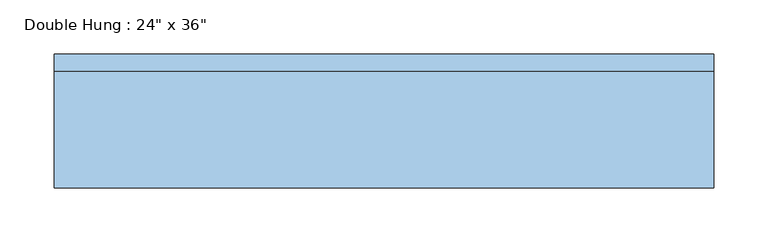
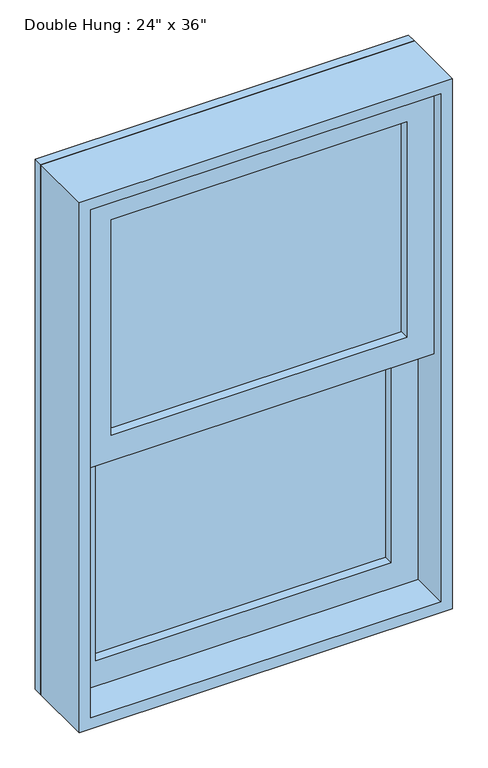
"""IFC4 building model written with IfcOpenShell, lengths in millimetres: window geometry."""

import ifcopenshell
import ifcopenshell.guid

model = None  # the IFC model being written
_history = None  # IfcOwnerHistory: only IFC2X3 demands one
_inside = {}  # id of a spatial element -> (the spatial element, [elements in it])
_under = {}  # id of a project, library or spatial element -> (it, [spatial elements below it])
_declared = {}  # id of a project -> (the project, [libraries it declares])
_typed = {}  # id of a type object -> (the type object, [elements of that type])
_made_of = {}  # id of a material, layer set ... -> (it, [elements and type objects made of it])


def new_model(schema):
    """Start an empty IFC model of exactly this schema.

    Asked for "IFC4X3", IfcOpenShell would pick the latest addendum, in which some entities
    have other attributes; the version numbers below select the first issue.
    IFC2X3 requires an IfcOwnerHistory on every rooted entity: one is made here for all.
    """
    global model, _history
    if schema == "IFC4X3":
        model = ifcopenshell.file(schema_version=(4, 3, 0, 0))
    else:
        model = ifcopenshell.file(schema=schema)
    _inside.clear()
    _under.clear()
    _declared.clear()
    _typed.clear()
    _made_of.clear()
    _history = None
    if model.schema == "IFC2X3":
        org = make("IfcOrganization", Name="unknown")
        user = make(
            "IfcPersonAndOrganization",
            ThePerson=make("IfcPerson", FamilyName="unknown"),
            TheOrganization=org,
        )
        app = make(
            "IfcApplication",
            ApplicationDeveloper=org,
            Version="unknown",
            ApplicationFullName="unknown",
            ApplicationIdentifier="unknown",
        )
        _history = make(
            "IfcOwnerHistory",
            OwningUser=user,
            OwningApplication=app,
            ChangeAction="ADDED",
            CreationDate=0,
        )
    return model


def make(cls, **values):
    """One entity of the class cls with the attributes given. An attribute that is None is left unset."""
    return model.create_entity(
        cls, **{name: value for name, value in values.items() if value is not None}
    )


def rooted(cls, **values):
    """An entity with a GlobalId (a new one), such as an element, a storey or a relation."""
    return make(cls, GlobalId=ifcopenshell.guid.new(), OwnerHistory=_history, **values)


def si_unit(unit_type, name, prefix=None):
    """IfcSIUnit, for example si_unit("LENGTHUNIT", "METRE", prefix="MILLI")."""
    return make("IfcSIUnit", UnitType=unit_type, Prefix=prefix, Name=name)


def assignment(units):
    """IfcUnitAssignment: the units of a project."""
    return None if units is None else make("IfcUnitAssignment", Units=units)


def point(xyz):
    """IfcCartesianPoint."""
    return None if xyz is None else make("IfcCartesianPoint", Coordinates=xyz)


def direction(xyz):
    """IfcDirection."""
    return None if xyz is None else make("IfcDirection", DirectionRatios=xyz)


def frame(location, z_axis=None, x_axis=None):
    """IfcAxis2Placement3D, a coordinate frame: its origin and axes. An axis left out is left unset."""
    return make(
        "IfcAxis2Placement3D",
        Location=point(location),
        Axis=direction(z_axis),
        RefDirection=direction(x_axis),
    )


def origin():
    """The frame at (0, 0, 0) with its axes left unset."""
    return frame((0.0, 0.0, 0.0))


def place(relative_to, where):
    """IfcLocalPlacement: puts the frame where relative to a parent placement (None: the world)."""
    return make(
        "IfcLocalPlacement", PlacementRelTo=relative_to, RelativePlacement=where
    )


def context(
    kind, dimensions, precision=None, world=None, true_north=None, identifier=None
):
    """IfcGeometricRepresentationContext, for example the 3D "Model" context."""
    return make(
        "IfcGeometricRepresentationContext",
        ContextIdentifier=identifier,
        ContextType=kind,
        CoordinateSpaceDimension=dimensions,
        Precision=precision,
        WorldCoordinateSystem=world,
        TrueNorth=true_north,
    )


def project(units=None, contexts=None):
    """IfcProject with its units and contexts."""
    return rooted(
        "IfcProject",
        Name="project",
        RepresentationContexts=contexts,
        UnitsInContext=assignment(units),
    )


def spatial(cls, under=None, at=None, **own):
    """A site, building, storey or space (cls), placed at a placement, below another one or the project."""
    s = rooted(cls, ObjectPlacement=at, **own)
    if under is not None:
        _under.setdefault(under.id(), (under, []))[1].append(s)
    return s


def polyline(points):
    """IfcPolyline through the points."""
    return make("IfcPolyline", Points=[point(p) for p in points])


def outline(outer, holes=None, kind="AREA"):
    """IfcArbitraryClosedProfileDef: a profile drawn as a closed curve; with holes, ...WithVoids."""
    if holes is None:
        return make("IfcArbitraryClosedProfileDef", ProfileType=kind, OuterCurve=outer)
    return make(
        "IfcArbitraryProfileDefWithVoids",
        ProfileType=kind,
        OuterCurve=outer,
        InnerCurves=holes,
    )


def extrude(swept, where, along, depth):
    """IfcExtrudedAreaSolid: the profile swept, set in the frame where, extruded along a direction by depth."""
    return make(
        "IfcExtrudedAreaSolid",
        SweptArea=swept,
        Position=where,
        ExtrudedDirection=direction(along),
        Depth=depth,
    )


def shape(context_of_items, identifier, shape_type, items):
    """IfcShapeRepresentation: the items that make up one representation, for example the "Body"."""
    return make(
        "IfcShapeRepresentation",
        ContextOfItems=context_of_items,
        RepresentationIdentifier=identifier,
        RepresentationType=shape_type,
        Items=items,
    )


def source(mapping_origin, context_of_items, identifier, shape_type, items):
    """IfcRepresentationMap: a shape defined once, which mapped items show again and again."""
    return make(
        "IfcRepresentationMap",
        MappingOrigin=mapping_origin,
        MappedRepresentation=shape(context_of_items, identifier, shape_type, items),
    )


def transform(
    local_origin,
    x_axis=None,
    y_axis=None,
    z_axis=None,
    scale=None,
    scale2=None,
    scale3=None,
    uniform=True,
):
    """IfcCartesianTransformationOperator3D, or its non-uniform kind. x_axis, y_axis, z_axis: its Axis1, 2, 3."""
    if uniform:
        return make(
            "IfcCartesianTransformationOperator3D",
            Axis1=direction(x_axis),
            Axis2=direction(y_axis),
            LocalOrigin=point(local_origin),
            Scale=scale,
            Axis3=direction(z_axis),
        )
    return make(
        "IfcCartesianTransformationOperator3DnonUniform",
        Axis1=direction(x_axis),
        Axis2=direction(y_axis),
        LocalOrigin=point(local_origin),
        Scale=scale,
        Axis3=direction(z_axis),
        Scale2=scale2,
        Scale3=scale3,
    )


def mapped(mapping_source, mapping_target):
    """IfcMappedItem: shows the shape of a source again, moved by a transform."""
    return make(
        "IfcMappedItem", MappingSource=mapping_source, MappingTarget=mapping_target
    )


def made_of(thing, what):
    """Note that an element or type object is made of a material, layer set ...; save() writes the relation."""
    if what is not None:
        _made_of.setdefault(what.id(), (what, []))[1].append(thing)
    return thing


def element(
    cls,
    number,
    at=None,
    inside=None,
    cuts=None,
    type_object=None,
    material=None,
    context=None,
    identifier="Body",
    shape_type=None,
    held_by="IfcProductDefinitionShape",
    body=None,
    shapes=None,
    **own,
):
    """One element of the class cls, such as IfcWall. Its Tag is "e" and its number.

    at: its placement. inside: the storey or other place that contains it. cuts: it is an
    opening in that element (IfcRelVoidsElement). A single representation is given by context,
    identifier, shape_type and body (its items); several are given by shapes. held_by: the class
    of the entity that holds the representations. save() writes the other relations.
    """
    e = rooted(cls, Tag="e%d" % number, ObjectPlacement=at, **own)
    if body is not None:
        shapes = [shape(context, identifier, shape_type, body)]
    if shapes is not None:
        e.Representation = make(held_by, Representations=shapes)
    if inside is not None:
        _inside.setdefault(inside.id(), (inside, []))[1].append(e)
    if cuts is not None:
        rooted(
            "IfcRelVoidsElement", RelatingBuildingElement=cuts, RelatedOpeningElement=e
        )
    if type_object is not None:
        _typed.setdefault(type_object.id(), (type_object, []))[1].append(e)
    return made_of(e, material)


def aggregate(whole, parts):
    """IfcRelAggregates: a whole, such as a stair, and the parts it consists of."""
    return rooted("IfcRelAggregates", RelatingObject=whole, RelatedObjects=parts)


def save(model, path):
    """Write the relations noted so far, then the file.

    IfcRelAggregates (storeys below a building ...), IfcRelContainedInSpatialStructure (elements
    in a storey), IfcRelDefinesByType, IfcRelAssociatesMaterial and IfcRelDeclares: one each for
    every whole, place, type object, material and project.
    """
    for whole, parts in _under.values():
        aggregate(whole, parts)
    for where, things in _inside.values():
        rooted(
            "IfcRelContainedInSpatialStructure",
            RelatedElements=things,
            RelatingStructure=where,
        )
    for kind, things in _typed.values():
        rooted("IfcRelDefinesByType", RelatedObjects=things, RelatingType=kind)
    for what, things in _made_of.values():
        rooted("IfcRelAssociatesMaterial", RelatedObjects=things, RelatingMaterial=what)
    for by, libraries in _declared.values():
        rooted("IfcRelDeclares", RelatingContext=by, RelatedDefinitions=libraries)
    model.write(path)


def window_9f7a67dd(model_context):
    return source(origin(), model_context, "Body", "SweptSolid", [
        extrude(outline(polyline([(-241.3, 17.4625), (-241.3, 30.1625), (241.3, 30.1625), (241.3, 17.4625), (-241.3, 17.4625)])), frame((0.0, 0.0, 977.9), z_axis=(0.0, 0.0, 1.0), x_axis=(1.0, 0.0, 0.0)), (0.0, 0.0, 1.0), 371.475),
        extrude(outline(polyline([(1393.825, -285.75), (933.45, -285.75), (933.45, 285.75), (1393.825, 285.75), (1393.825, -285.75)]), holes=[polyline([(1349.375, -241.3), (1349.375, 241.3), (977.9, 241.3), (977.9, -241.3), (1349.375, -241.3)])]), frame((0.0, 1.5875, 0.0), z_axis=(0.0, 1.0, 0.0), x_axis=(0.0, 0.0, 1.0)), (0.0, 0.0, 1.0), 44.45),
        extrude(outline(polyline([(241.3, -14.2875), (241.3, -26.9875), (-241.3, -26.9875), (-241.3, -14.2875), (241.3, -14.2875)])), frame((0.0, 0.0, 1393.825), z_axis=(0.0, 0.0, 1.0), x_axis=(1.0, 0.0, 0.0)), (0.0, 0.0, 1.0), 371.475),
        extrude(outline(polyline([(1809.75, -285.75), (1349.375, -285.75), (1349.375, 285.75), (1809.75, 285.75), (1809.75, -285.75)]), holes=[polyline([(1765.3, -241.3), (1765.3, 241.3), (1393.825, 241.3), (1393.825, -241.3), (1765.3, -241.3)])]), frame((0.0, -42.8625, 0.0), z_axis=(0.0, 1.0, 0.0), x_axis=(0.0, 0.0, 1.0)), (0.0, 0.0, 1.0), 44.45),
        extrude(outline(polyline([(1828.8, -304.8), (914.4, -304.8), (914.4, 304.8), (1828.8, 304.8), (1828.8, -304.8)]), holes=[polyline([(1797.05, -273.05), (1797.05, 273.05), (946.15, 273.05), (946.15, -273.05), (1797.05, -273.05)])]), frame((0.0, 46.0375, 0.0), z_axis=(0.0, 1.0, 0.0), x_axis=(0.0, 0.0, 1.0)), (0.0, 0.0, 1.0), 15.875),
        extrude(outline(polyline([(1828.8, 304.8), (1828.8, -304.8), (914.4, -304.8), (914.4, 304.8), (1828.8, 304.8)]), holes=[polyline([(1809.75, 285.75), (933.45, 285.75), (933.45, -285.75), (1809.75, -285.75), (1809.75, 285.75)])]), frame((0.0, -61.9125, 0.0), z_axis=(0.0, 1.0, 0.0), x_axis=(0.0, 0.0, 1.0)), (0.0, 0.0, 1.0), 107.95),
    ])


if __name__ == "__main__":
    model = new_model("IFC4")
    model_context = context("Model", 3, world=origin())
    ifc_project = project(units=[si_unit("LENGTHUNIT", "METRE", prefix="MILLI")], contexts=[model_context])
    site = spatial("IfcSite", under=ifc_project)
    building = spatial("IfcBuilding", under=site)
    placement = place(None, origin())
    window_shape = window_9f7a67dd(model_context)
    element("IfcWindow", 1, ObjectType="Double Hung : 24\" x 36\"", at=placement, inside=building, context=model_context, shape_type="MappedRepresentation", body=[
        mapped(window_shape, transform((0.0, 0.0, 0.0), x_axis=(1.0, 0.0, 0.0), y_axis=(0.0, 1.0, 0.0), z_axis=(0.0, 0.0, 1.0))),
    ])
    save(model, "model.ifc")

# Revit data of these elements
# Project information
#   Sheets - Total = "6"
#   Project Issue Date = "Issue Date"
#   Project Status = "Project Status"
#   Client Name = "Owner"
#   Project Address = "Enter address here"
#   Project Name = "Project Name"
#   Project Number = "Project Number"
#   Publication Date = "30-Jan-15"
# Type "Double Hung : 24\" x 36\""
#   Type Mark = "19"
#   Assembly Code = "B2020100"
#   Height = 3' - 0"
#   Default Sill Height = 3' - 0"
#   Width = 2' - 0"
#   Window Inset = 0' - 0 3/4"
#   Glass Pane Material = Glass
#   Sash Material = Sash
#   Description = (empty or 0)
#   Wall Closure = (empty or 0)
# Element 1 (IfcWindow, "Double Hung : 24\" x 36\"")
#   Materials on its faces: "Sash", "Glass"
# Materials
#   "Glass": class "Glass", colour RGB 0 128 192, transparency 0.75
#   "Sash": class "Wood", colour RGB 224 178 126, transparency 0
